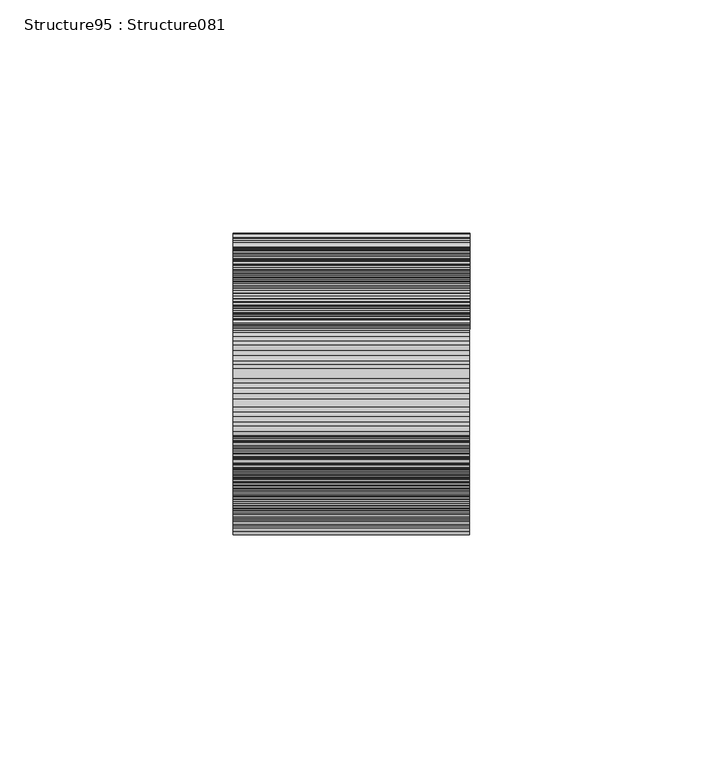
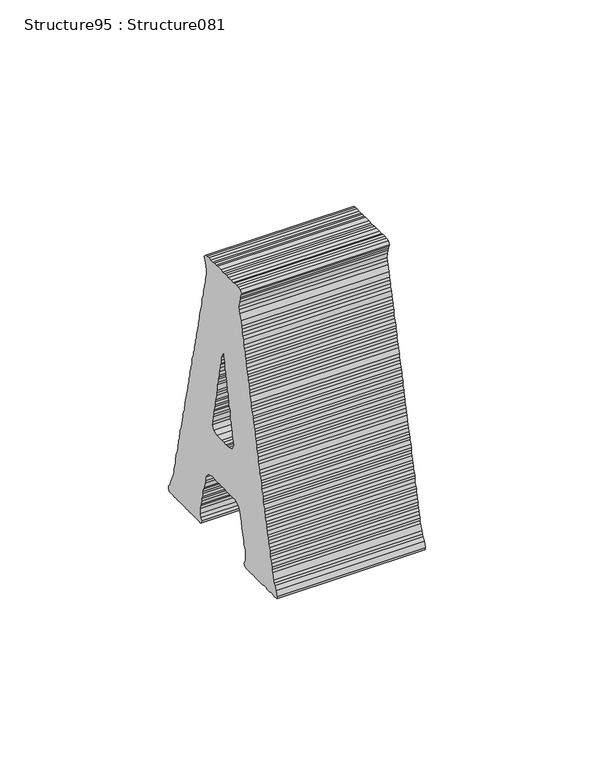
"""IFC4 building model written with IfcOpenShell, lengths in millimetres: proxy geometry, Structure95 : Structure081."""

from ifc_helpers import new_model, si_unit, frame, origin, place, context, project, spatial, polyline, outline, extrude, source, transform, mapped, element, save


def structure95_structure081_7d0c17b7(model_context):
    return source(origin(), model_context, "Body", "SweptSolid", [
        extrude(outline(polyline([(0.9094651, 0.0), (2.0811665, -0.5212702), (2.9906316, -0.6507871), (4.1562841, -0.780304), (5.1991801, -1.1720572), (5.9748585, -1.3012183), (7.1504738, -1.6890575), (8.1894559, -1.6890575), (9.3551083, -2.0808107), (10.2645735, -2.3398446), (11.4362748, -2.5981668), (12.3453841, -2.8611147), (13.3818755, -2.9902758), (14.1582655, -3.378115), (15.4626861, -3.509411), (16.3721513, -3.509411), (17.5385154, -3.7698682), (19.491944, -4.4188762), (20.2718921, -4.6793333), (21.3101626, -4.9383671), (22.3470097, -4.9383671), (23.2561191, -5.1988244), (24.4278204, -5.5866635), (25.4700048, -5.9766376), (26.6363689, -5.9766376), (27.4124031, -6.3666117), (28.7175354, -6.6274246), (30.535754, -7.0173988), (31.5743802, -7.148339), (32.7400327, -7.4073728), (33.6555467, -7.7969911), (35.4741211, -7.7969911), (36.5102567, -7.5361781), (37.5492387, -7.275721), (38.3288311, -6.8878818), (39.3671015, -6.3666117), (40.4099976, -7.275721), (40.5395145, -8.1851861), (40.5395145, -9.0964303), (40.2826155, -10.2659968), (40.2826155, -11.3042672), (40.5395145, -12.4745453), (40.4099976, -13.2523585), (40.5395145, -14.1639586), (40.5395145, -16.2429902), (40.2826155, -17.2791257), (40.2826155, -18.3198869), (40.5395145, -19.4915882), (40.4099976, -20.6575965), (40.4099976, -22.346654), (40.2826155, -23.5183553), (40.5395145, -24.4274646), (40.5395145, -25.595252), (40.4099976, -26.5047172), (40.2826155, -27.6742836), (39.2382962, -28.4545876), (38.3288311, -27.9372314), (37.4197218, -27.6742836), (36.6397736, -27.5454783), (35.4741211, -27.2846653), (33.5199809, -26.8964703), (32.6112274, -27.157639), (31.4448633, -27.4138265), (29.3636968, -28.1937747), (27.545834, -28.4545876), (26.5089869, -28.7150447), (25.3372855, -28.8445616), (24.2943895, -29.1032398), (23.2561191, -29.6262889), (21.3101626, -29.7540268), (20.2718921, -30.0144839), (19.491944, -30.5336191), (18.3202426, -30.5336191), (17.2816164, -30.9235932), (16.3721513, -31.1840504), (15.3356599, -31.1840504), (14.1582655, -31.4427284), (13.1253323, -31.8330583), (12.2158672, -32.2230325), (11.4362748, -32.3518378), (10.2645735, -32.4834896), (9.3551083, -32.8731079), (8.1894559, -32.8731079), (7.1504738, -33.2613029), (6.2374505, -33.3925989), (5.0714422, -33.653056), (3.2475306, -34.302064), (2.0811665, -34.302064), (1.1720572, -34.5625211), (0.1334309, -34.8208434), (-1.0382704, -35.3421135), (-1.8178628, -35.4716304), (-2.8568449, -35.7303086), (-3.8990293, -35.8616046), (-5.0653934, -36.2515786), (-5.8471206, -36.5099009), (-7.0166871, -36.5099009), (-8.1826954, -36.899875), (-8.9644226, -37.0315268), (-10.1364798, -37.4193661), (-11.1690572, -37.5506621), (-12.2115974, -37.680179), (-12.9915456, -37.9406361), (-14.03373, -38.3284753), (-15.3292552, -38.4601272), (-16.3678815, -38.7205843), (-18.1861001, -39.1084235), (-19.3581573, -39.3692365), (-20.2672666, -39.7574315), (-21.4371888, -40.0178886), (-22.2189161, -40.2783458), (-23.1223323, -40.5370239), (-24.1648726, -40.5370239), (-25.465735, -41.0586497), (-26.5025822, -41.316972), (-27.4173846, -41.446489), (-28.4560108, -41.446489), (-29.235959, -41.7069461), (-30.5311284, -42.0986993), (-31.3110766, -42.2264372), (-32.3536168, -42.6181903), (-33.5214042, -42.6181903), (-34.4308693, -43.1355465), (-35.3399786, -43.3960036), (-36.37647, -43.3960036), (-37.5424783, -43.6564607), (-38.7202285, -44.0443), (-39.6236447, -44.3072478), (-40.405372, -44.5659258), (-41.5752942, -44.695087), (-42.6139205, -45.0850611), (-43.7856218, -45.3455182), (-44.8221132, -45.3455182), (-45.7372714, -45.4732561), (-46.6406876, -45.9963053), (-47.812389, -46.2549833), (-48.8510152, -46.5140172), (-49.7601245, -46.5140172), (-50.6731478, -46.9057704), (-52.8777823, -47.5540667), (-53.7929405, -47.9419059), (-54.5689747, -48.3340149), (-55.738897, -49.1118282), (-57.5532016, -49.7626153), (-58.4665807, -49.5035814), (-58.5957419, -48.2030747), (-58.4665807, -47.4227707), (-58.3331498, -46.2549833), (-58.5957419, -45.2167129), (-58.5957419, -44.0443), (-58.3331498, -43.0060296), (-58.3331498, -42.0986993), (-58.4665807, -41.0586497), (-58.4665807, -40.1491846), (-58.5957419, -38.8479664), (-58.5957419, -37.9406361), (-58.4665807, -36.899875), (-58.3331498, -35.7303086), (-58.5957419, -34.8208434), (-58.5957419, -31.8330583), (-58.3331498, -30.6627802), (-57.4297336, -30.1440009), (-56.6480063, -30.5336191), (-55.6115149, -30.7940763), (-53.3972734, -30.7940763), (-52.3586471, -30.7940763), (-51.4495378, -30.5336191), (-50.6731478, -30.1440009), (-49.3683714, -30.0144839), (-48.4592621, -29.7540268), (-47.5497969, -29.3636969), (-46.6406876, -29.1032398), (-45.6038405, -28.8445616), (-43.2661308, -28.5855278), (-41.5752942, -27.9372314), (-40.2762109, -27.6742836), (-38.9767716, -27.0259872), (-38.1950444, -26.1168779), (-37.4190102, -24.6864985), (-37.6759092, -23.6478723), (-37.6759092, -21.5688407), (-37.5424783, -20.2694015), (-37.5424783, -17.5420736), (-37.6759092, -16.3700164), (-37.4190102, -15.463042), (-37.5424783, -14.42406), (-37.6759092, -13.3840104), (-37.5424783, -12.4745453), (-37.4190102, -11.1754619), (-37.6759092, -10.3955137), (-38.0676623, -8.8373965), (-38.8476105, -8.0556692), (-40.2762109, -7.0173988), (-41.4422191, -7.0173988), (-42.6139205, -6.7562299), (-44.561656, -6.2388739), (-45.3472973, -5.7179595), (-46.5133056, -5.4592815), (-47.2932538, -5.3283413), (-48.33188, -5.3283413), (-49.3683714, -4.8067153), (-50.4126907, -4.6793333), (-51.4495378, -4.5501722), (-52.3586471, -4.158419), (-53.6595096, -3.7698682), (-55.3489229, -3.897606), (-56.6480063, -4.2875802), (-57.2966585, -4.9383671), (-58.5957419, -4.158419), (-58.4665807, -2.9902758), (-58.3331498, -1.9498705), (-58.3331498, 0.1291611), (-58.4665807, 1.1677873), (-58.4665807, 2.2060577), (-58.3331498, 3.1176577), (-58.4665807, 4.0267671), (-58.4665807, 5.3258505), (-58.3331498, 6.1040196), (-58.4665807, 7.4052379), (-58.3331498, 8.1848303), (-58.5957419, 9.2252356), (-58.3331498, 10.3933787), (-58.5957419, 11.5633011), (-58.4665807, 12.4724104), (-58.3331498, 13.5128157), (-58.3331498, 14.5496629), (-57.2966585, 14.941416), (-56.3875492, 14.6809589), (-55.738897, 14.0301718), (-54.5689747, 13.7718495), (-53.7929405, 13.3818754), (-52.6151903, 12.8602495), (-50.6731478, 11.9511402), (-49.8875066, 11.692818), (-48.5941162, 11.5633011), (-47.5497969, 11.3028439), (-46.6406876, 11.04381), (-45.8646534, 10.6520569), (-44.5616561, 10.5225398), (-42.6139205, 10.2638618), (-41.4422191, 9.8738878), (-40.5384471, 9.4821345), (-39.6236447, 9.2252356), (-38.4576364, 9.0942954), (-37.4190102, 8.9626436), (-36.5059869, 8.8338383), (-35.6004358, 8.3143472), (-34.2956593, 8.1848303), (-33.3922431, 8.0535342), (-32.3536168, 7.9243731), (-31.4405935, 7.5365339), (-30.4019673, 7.1447808), (-29.235959, 6.8857468), (-27.5447666, 6.6252897), (-26.3752002, 6.2353156), (-25.203143, 6.1040196), (-24.4235506, 5.8474764), (-23.3849244, 5.4553674), (-22.4793732, 5.3258505), (-21.3037579, 4.9362322), (-20.2672666, 4.9362322), (-19.3581573, 4.6750634), (-18.319531, 4.4167412), (-17.1474738, 4.158419), (-15.2018732, 3.636793), (-14.1632469, 3.3777592), (-13.1207067, 3.3777592), (-12.2115974, 2.9860059), (-11.3024881, 2.5981668), (-10.0012698, 2.5981668), (-9.2270147, 2.0772524), (-8.1826954, 2.0772524), (-7.0166871, 1.9498704), (-5.9745027, 1.4282445), (-5.0653934, 1.4282445), (-4.1619771, 0.9091093), (-2.8568449, 0.7799482), (-1.9473797, 0.7799482), (-0.7817273, 0.2604571), (0.0, 0.0), (0.9094651, 0.0)]), holes=[polyline([(-20.9137838, -13.9010107), (-20.9137838, -16.8912865), (-20.7903157, -18.0590739), (-21.0472147, -19.2311311), (-20.7903157, -20.1398846), (-20.9137838, -21.0493497), (-20.2672666, -22.997441), (-18.5817672, -23.6478723), (-17.2809048, -23.3874151), (-16.3678815, -23.1262463), (-15.4623303, -22.870059), (-14.1632469, -22.997441), (-13.2480888, -22.47795), (-12.2115974, -22.346654), (-11.3024881, -22.2174928), (-10.393023, -21.8292979), (-9.3508386, -21.6983576), (-8.3122123, -21.6983576), (-7.146204, -21.5688407), (-6.3644768, -21.1806457), (-5.3276296, -20.9201886), (-4.2854452, -20.9201886), (-3.117302, -20.4010533), (-1.9473797, -20.4010533), (-1.0382704, -20.0089444), (-0.2561874, -19.8794274), (1.0389821, -19.7481313), (2.0811665, -19.4915882), (3.1180136, -19.2311311), (4.0274787, -19.0998351), (5.0714422, -19.0998351), (6.1082894, -18.580344), (7.0177545, -18.4508271), (8.1894559, -18.4508271), (9.2216774, -18.0590739), (10.1368356, -17.8025307), (11.0463007, -17.8025307), (10.1368356, -17.1520995), (9.0928721, -16.7617696), (8.056025, -16.6308294), (6.8900167, -16.6308294), (6.1082894, -16.1134732), (4.9365881, -15.9818214), (3.1180136, -15.463042), (1.8189302, -15.3335251), (0.9094651, -15.202229), (0.0, -14.9417719), (-1.0382704, -14.8122549), (-2.2078369, -14.42406), (-4.2854452, -14.2927639), (-5.3276296, -14.0323067), (-6.3644768, -13.9010107), (-8.1826954, -13.5128158), (-9.2270147, -12.9936805), (-10.2638619, -12.9936805), (-11.1690572, -12.7332234), (-12.3446725, -12.6037065), (-13.1207067, -12.2115974), (-14.286715, -12.2115974), (-15.4623303, -11.8237583), (-17.2809048, -11.5633011), (-18.5817672, -11.3042672), (-20.1377496, -12.0845712), (-20.9137838, -13.9010107)])]), frame((-56111.3037332, 291733.8164793, -317.0048136), z_axis=(-0.9999998917542984, 0.00046528635450596156, 0.0), x_axis=(0.0, 0.0, 1.0)), (0.0, 0.0, 1.0), 50.8),
    ])


if __name__ == "__main__":
    model = new_model("IFC4")
    model_context = context("Model", 3, world=origin())
    ifc_project = project(units=[si_unit("LENGTHUNIT", "METRE", prefix="MILLI")], contexts=[model_context])
    site = spatial("IfcSite", under=ifc_project)
    building = spatial("IfcBuilding", under=site)
    placement = place(None, origin())
    structure95_structure081_shape = structure95_structure081_7d0c17b7(model_context)
    element("IfcBuildingElementProxy", 1, Name="Structure95 : Structure081", ObjectType="Structure95 : Structure081", at=placement, inside=building, context=model_context, shape_type="MappedRepresentation", body=[
        mapped(structure95_structure081_shape, transform((0.0, 0.0, 0.0), x_axis=(1.0, 0.0, 0.0), y_axis=(0.0, 1.0, 0.0), z_axis=(0.0, 0.0, 1.0))),
    ])
    save(model, "model.ifc")

# Revit data of these elements
# Type "Structure95 : Structure081"
#   NameOverride = "Structure081"
# Element 1 (IfcBuildingElementProxy, "Structure95 : Structure081")
#   Materials on its faces: "BRUSHED ALUMINUM LETTERING"
# Materials
#   "BRUSHED ALUMINUM LETTERING": class "Unassigned", colour RGB 169 181 186, transparency 0, Cost = 0
